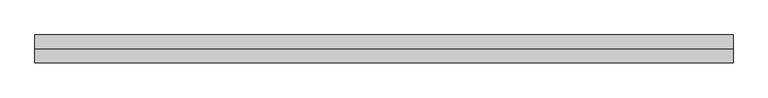
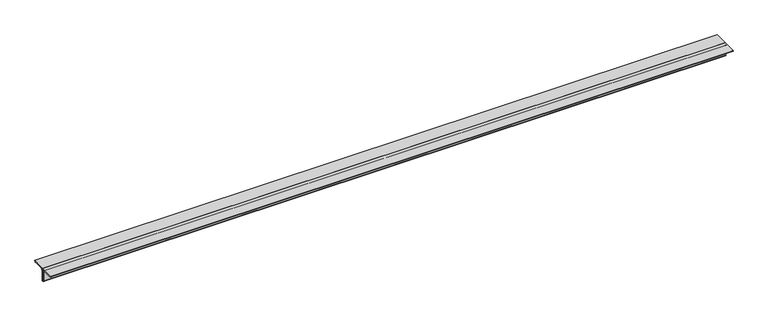
"""IFC4 building model written with IfcOpenShell, lengths in millimetres: member geometry, Steel Framing_2Ls_KS : H_SB_AR_S02_2Ls-100x100x10_VBR1."""

from ifc_helpers import new_model, si_unit, point, frame, frame_2d, origin, place, context, project, spatial, polyline, circle_curve, trimmed, segment, composite_curve, outline, extrude, source, transform, mapped, element, save


def member_f7a1a9e2(model_context):
    return source(origin(), model_context, "Body", "SweptSolid", [
        extrude(outline(composite_curve([segment(polyline([(0.0, 28.2), (100.0, 28.2)]), True, "CONTINUOUS"), segment(trimmed(circle_curve(frame_2d((90.0, 28.2)), 10.0), [point((100.0, 28.2))], [point((90.0, 18.2))], False, "CARTESIAN"), True, "CONTINUOUS"), segment(polyline([(90.0, 18.2), (20.0, 18.2)]), True, "CONTINUOUS"), segment(trimmed(circle_curve(frame_2d((20.0, 8.2)), 10.0), [point((20.0, 18.2))], [point((10.0, 8.2))], True, "CARTESIAN"), True, "CONTINUOUS"), segment(polyline([(10.0, 8.2), (10.0, -61.8)]), True, "CONTINUOUS"), segment(trimmed(circle_curve(frame_2d((0.0, -61.8)), 10.0), [point((10.0, -61.8))], [point((0.0, -71.8))], False, "CARTESIAN"), True, "CONTINUOUS"), segment(polyline([(0.0, -71.8), (0.0, 28.2)]), True, "CONTINUOUS")], self_intersect=False)), frame((-2391.9159074, 0.0, 0.0), z_axis=(1.0, 0.0, 0.0), x_axis=(0.0, 1.0, 0.0)), (0.0, 0.0, 1.0), 4992.4085104),
        extrude(outline(composite_curve([segment(polyline([(0.0, 28.2), (0.0, -71.8)]), True, "CONTINUOUS"), segment(trimmed(circle_curve(frame_2d((0.0, -61.8)), 10.0), [point((0.0, -71.8))], [point((-10.0, -61.8))], False, "CARTESIAN"), True, "CONTINUOUS"), segment(polyline([(-10.0, -61.8), (-10.0, 8.2)]), True, "CONTINUOUS"), segment(trimmed(circle_curve(frame_2d((-20.0, 8.2)), 10.0), [point((-10.0, 8.2))], [point((-20.0, 18.2))], True, "CARTESIAN"), True, "CONTINUOUS"), segment(polyline([(-20.0, 18.2), (-90.0, 18.2)]), True, "CONTINUOUS"), segment(trimmed(circle_curve(frame_2d((-90.0, 28.2)), 10.0), [point((-90.0, 18.2))], [point((-100.0, 28.2))], False, "CARTESIAN"), True, "CONTINUOUS"), segment(polyline([(-100.0, 28.2), (0.0, 28.2)]), True, "CONTINUOUS")], self_intersect=False)), frame((-2391.9159074, 0.0, 0.0), z_axis=(1.0, 0.0, 0.0), x_axis=(0.0, 1.0, 0.0)), (0.0, 0.0, 1.0), 4992.4085104),
    ])


if __name__ == "__main__":
    model = new_model("IFC4")
    model_context = context("Model", 3, world=origin())
    ifc_project = project(units=[si_unit("LENGTHUNIT", "METRE", prefix="MILLI")], contexts=[model_context])
    site = spatial("IfcSite", under=ifc_project)
    building = spatial("IfcBuilding", under=site)
    placement = place(None, origin())
    member_shape = member_f7a1a9e2(model_context)
    element("IfcMember", 1, ObjectType="Steel Framing_2Ls_KS : H_SB_AR_S02_2Ls-100x100x10_VBR1", at=placement, inside=building, context=model_context, shape_type="MappedRepresentation", body=[
        mapped(member_shape, transform((0.0, 0.0, 0.0), x_axis=(1.0, 0.0, 0.0), y_axis=(0.0, 1.0, 0.0), z_axis=(0.0, 0.0, 1.0))),
    ])
    save(model, "model.ifc")

# Revit data of these elements
# Type "Steel Framing_2Ls_KS : H_SB_AR_S02_2Ls-100x100x10_VBR1"
#   Type Comments = "MAIN"
#   Type Mark = "VBR1"
#   H_SectionID = "2Ls-100x100x10"
#   Assembly Code = "B10"
#   Legs = "LLBB"
#   H_Ratio for Additional Steel Plate = 0.2
#   W = 0
#   Perimeter = 0.80 m²/m
#   Nominal Weight = 29.80 kgf/m
#   Length [instance default] = 1524 mm
#   Space = 0 mm
#   b = 100 mm
#   d = 100 mm
#   t = 10 mm
#   y = 28.2 mm
#   A = 0.0038 m²
#   Structural Material [instance default] = Steel, 45-345
# Element 1 (IfcMember, "Steel Framing_2Ls_KS : H_SB_AR_S02_2Ls-100x100x10_VBR1")
#   Materials on its faces: "Steel, 45-345"
# Materials
#   "Steel, 45-345": class "Metal", colour RGB 189 187 185, transparency 0, Description = "Steel 345 MPa", Cost = 0
